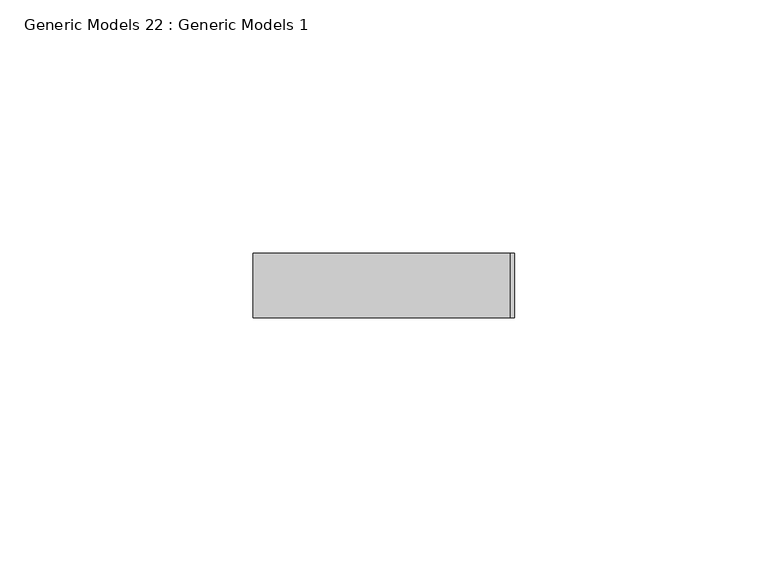
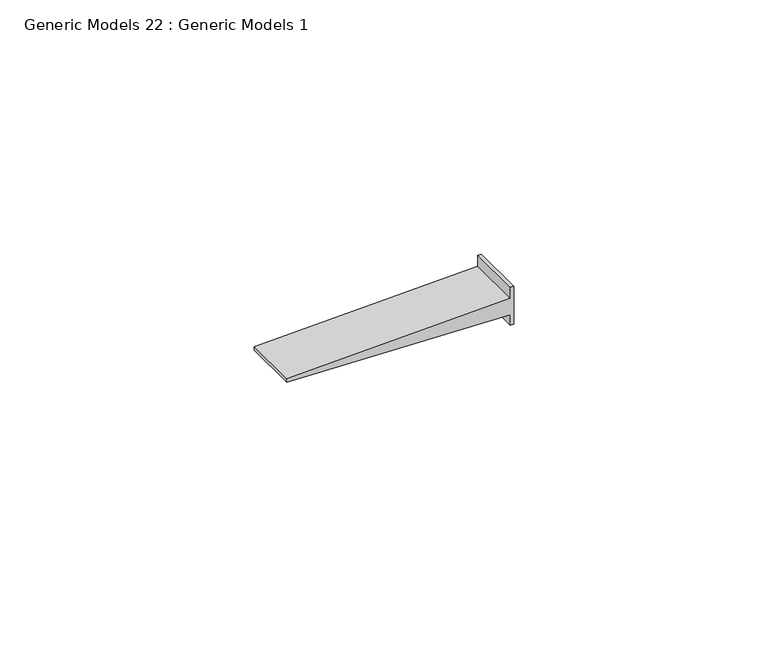
"""IFC4 building model written with IfcOpenShell, lengths in millimetres: proxy geometry, Generic Models 22 : Generic Models 1."""

from ifc_helpers import new_model, si_unit, frame, origin, place, context, project, spatial, polyline, outline, extrude, source, transform, mapped, element, save


def generic_models_22_generic_models_1_e5767157(model_context):
    return source(origin(), model_context, "Body", "SweptSolid", [
        extrude(outline(polyline([(2409.6091, 49800.66875), (2409.6091, 49799.875), (2407.0592364, 49799.875), (2405.4618473, 49749.075), (2404.6631527, 49749.075), (2403.0657636, 49799.875), (2400.5159, 49799.875), (2400.5159, 49800.66875), (2409.6091, 49800.66875)])), frame((0.0, 565.15, 0.0), z_axis=(0.0, 1.0, 0.0), x_axis=(0.0, 0.0, 1.0)), (0.0, 0.0, 1.0), 12.7),
    ])


if __name__ == "__main__":
    model = new_model("IFC4")
    model_context = context("Model", 3, world=origin())
    ifc_project = project(units=[si_unit("LENGTHUNIT", "METRE", prefix="MILLI")], contexts=[model_context])
    site = spatial("IfcSite", under=ifc_project)
    building = spatial("IfcBuilding", under=site)
    placement = place(None, origin())
    generic_models_22_generic_models_1_shape = generic_models_22_generic_models_1_e5767157(model_context)
    element("IfcBuildingElementProxy", 1, Name="Generic Models 22 : Generic Models 1", ObjectType="Generic Models 22 : Generic Models 1", at=placement, inside=building, context=model_context, shape_type="MappedRepresentation", body=[
        mapped(generic_models_22_generic_models_1_shape, transform((0.0, 0.0, 0.0), x_axis=(1.0, 0.0, 0.0), y_axis=(0.0, 1.0, 0.0), z_axis=(0.0, 0.0, 1.0))),
    ])
    save(model, "model.ifc")

# Revit data of these elements
# Element 1 (IfcBuildingElementProxy, "Generic Models 22 : Generic Models 1")
#   Materials on its faces: "ATTACH GYPSUM BOARD TO STUDS AND NOT TO TOP TRACK"
# Materials
#   "ATTACH GYPSUM BOARD TO STUDS AND NOT TO TOP TRACK": class "Generic", colour RGB 48 48 48, transparency 0, Cost = 0
